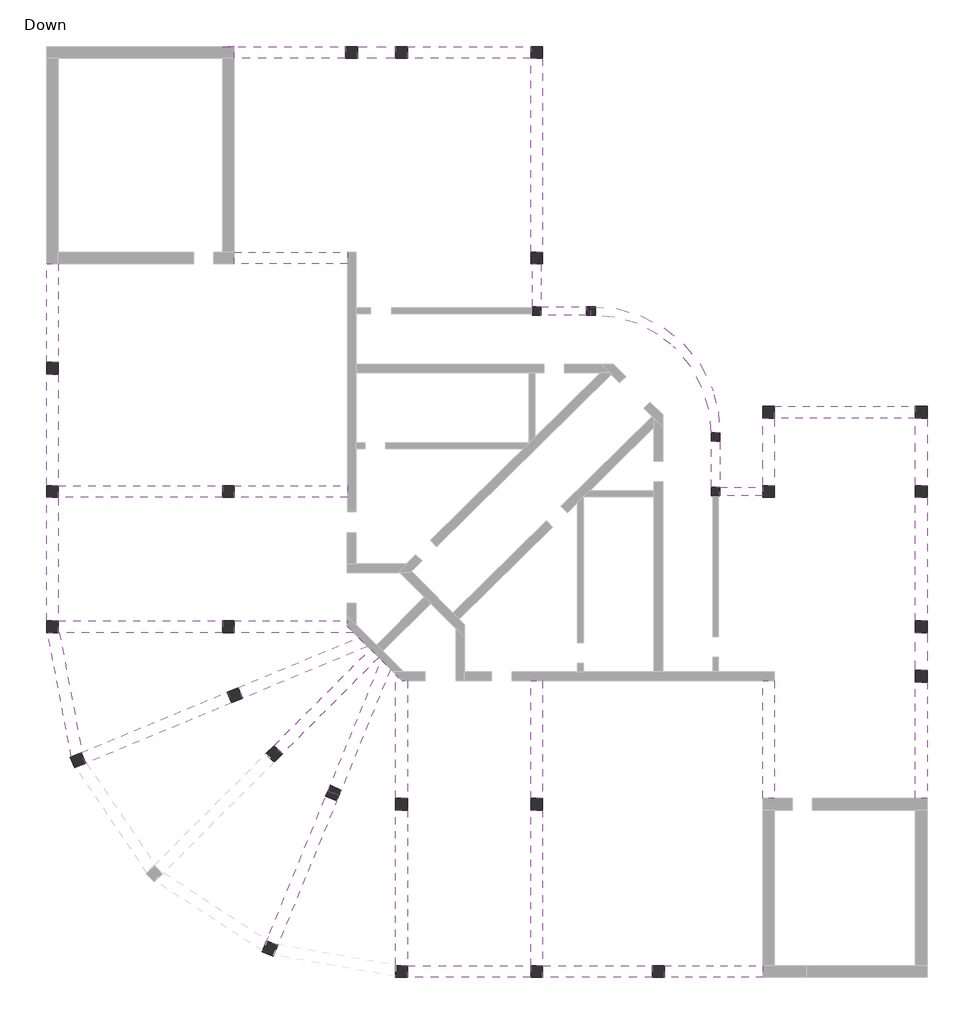
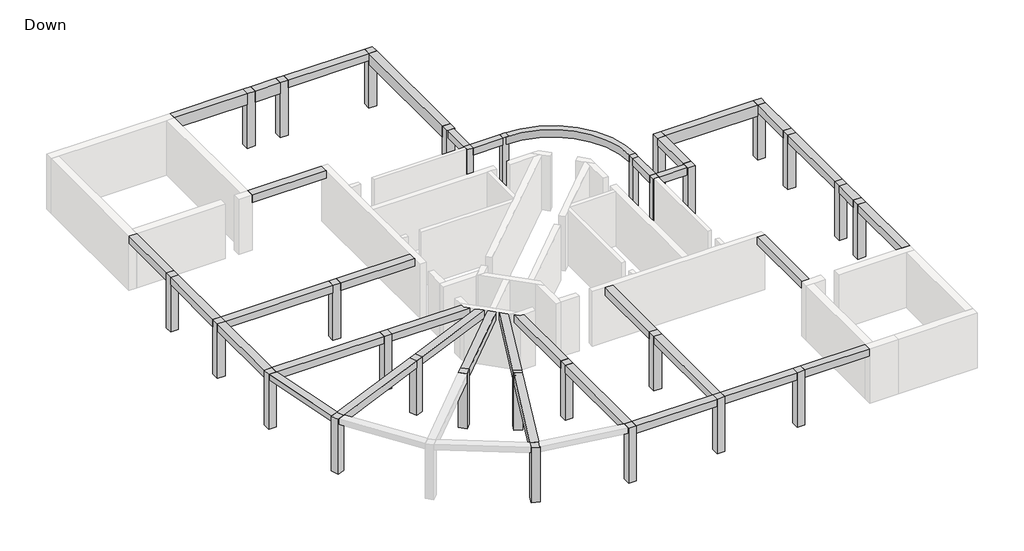
# One storey, part 2 of 2: 37 beams, 29 columns.
"""IFC4 building model written with IfcOpenShell, lengths in millimetres."""

from ifc_helpers import new_model, si_unit, point, frame, frame_2d, origin, origin_with_axes, place, context, project, spatial, polyline, circle_curve, trimmed, segment, composite_curve, outline, extrude, faceted_brep, element, save

model = new_model("IFC4")

# Units and contexts
model_context = context("Model", 3, world=origin())
ifc_project = project(units=[si_unit("LENGTHUNIT", "METRE", prefix="MILLI")], contexts=[model_context])

# Site, building, storey
site = spatial("IfcSite", under=ifc_project)
building = spatial("IfcBuilding", under=site)
storey = spatial("IfcBuildingStorey", under=building, Name="Down", Elevation=0.0)

# Beams
placement = place(None, origin())
element("IfcBeam", 1, ObjectType="Concrete Rectengular Beam : 30/40", at=placement, inside=storey, context=model_context, shape_type="Brep", body=[
    faceted_brep([(9669.6339123, 9562.1590026, 3000.0), (9669.6339123, 9862.1590026, 3000.0), (8219.6339123, 9862.1590026, 3000.0), (8219.6339123, 9562.1590026, 3000.0), (9669.6339123, 9862.1590026, 2600.0), (8219.6339123, 9862.1590026, 2600.0), (9669.6339123, 9562.1590026, 2600.0), (8219.6339123, 9562.1590026, 2600.0), (8219.6339123, 9562.1590026, 2800.0), (9669.6339123, 9562.1590026, 2800.0)], [[[0, 1, 2, 3]], [[1, 4, 5, 2]], [[4, 6, 7, 5]], [[0, 3, 8, 7, 6, 9]], [[4, 1, 0, 9, 6]], [[3, 2, 5, 7, 8]]]),
])
element("IfcBeam", 2, ObjectType="Concrete Rectengular Beam : 30/40", at=placement, inside=storey, context=model_context, shape_type="Brep", body=[
    faceted_brep([(7919.6339123, 9862.1590026, 3000.0), (8219.6339123, 9862.1590026, 3000.0), (8219.6339123, 11415.5910733, 3000.0), (7919.6339123, 11415.5910733, 3000.0), (8219.6339123, 9862.1590026, 2600.0), (8219.6339123, 11415.5910733, 2600.0), (7919.6339123, 9862.1590026, 2600.0), (7919.6339123, 11415.5910733, 2600.0), (7919.6339123, 11415.5910733, 2800.0), (7919.6339123, 9862.1590026, 2800.0)], [[[0, 1, 2, 3]], [[1, 4, 5, 2]], [[4, 6, 7, 5]], [[0, 3, 8, 7, 6, 9]], [[4, 1, 0, 9, 6]], [[3, 2, 5, 7, 8]]]),
])
element("IfcBeam", 3, ObjectType="Concrete Rectengular Beam : 30/40", at=placement, inside=storey, context=model_context, shape_type="SweptSolid", body=[
    extrude(outline(composite_curve([segment(polyline([(3827.8442558, 15704.0519912), (3819.9226923, 16003.9473877)]), True, "CONTINUOUS"), segment(trimmed(circle_curve(frame_2d((3933.1798389, 11716.2462427)), 4289.1966953), [point((3819.9226923, 16003.9473877))], [point((8219.6339123, 11562.8846875))], False, "CARTESIAN"), True, "CONTINUOUS"), segment(polyline([(8219.6339123, 11562.8846875), (8219.6339123, 11715.5910733), (7922.3764803, 11715.5910733)]), True, "CONTINUOUS"), segment(trimmed(circle_curve(frame_2d((3933.1798389, 11716.2462427)), 3989.1966953), [point((7922.3764803, 11715.5910733))], [point((3827.8442558, 15704.0519912))], True, "CARTESIAN"), True, "CONTINUOUS")], self_intersect=False)), frame((0.0, 0.0, 2600.0), z_axis=(0.0, 0.0, 1.0), x_axis=(1.0, 0.0, 0.0)), (0.0, 0.0, 1.0), 400.0),
])
element("IfcBeam", 4, ObjectType="Concrete Rectengular Beam : 30/40", at=placement, inside=storey, context=model_context, shape_type="Brep", body=[
    faceted_brep([(2129.020722, 16003.9996895, 3000.0), (2129.020722, 15703.9996895, 3000.0), (3673.883474, 15703.9996895, 3000.0), (3673.883474, 16003.9996895, 3000.0), (2129.020722, 16003.9996895, 2600.0), (3673.883474, 16003.9996895, 2600.0), (2129.020722, 15703.9996895, 2600.0), (3673.883474, 15703.9996895, 2600.0), (2129.020722, 15703.9996895, 2800.0), (3673.883474, 15703.9996895, 2800.0)], [[[0, 1, 2, 3]], [[4, 0, 3, 5]], [[6, 4, 5, 7]], [[2, 1, 8, 6, 7, 9]], [[1, 0, 4, 6, 8]], [[3, 2, 9, 7, 5]]]),
])
element("IfcBeam", 5, ObjectType="Concrete Rectengular Beam : 30/40", at=placement, inside=storey, context=model_context, shape_type="Brep", body=[
    faceted_brep([(2129.020722, 17453.6134053, 3000.0), (1829.020722, 17453.6134053, 3000.0), (1829.020722, 16003.9996895, 3000.0), (2129.020722, 16003.9996895, 3000.0), (2129.020722, 17453.6134053, 2600.0), (2129.020722, 16003.9996895, 2600.0), (1829.020722, 17453.6134053, 2600.0), (1829.020722, 16003.9996895, 2600.0), (1829.020722, 17453.6134053, 2800.0)], [[[0, 1, 2, 3]], [[4, 0, 3, 5]], [[6, 4, 5, 7]], [[1, 8, 6, 7, 2]], [[1, 0, 4, 6, 8]], [[2, 7, 5, 3]]]),
])
element("IfcBeam", 6, ObjectType="Concrete Rectengular Beam : 39/30", at=placement, inside=storey, context=model_context, shape_type="Brep", body=[
    faceted_brep([(-13852.0238981, 697.9157956, 3000.0), (-13520.7080657, 835.1736918, 3000.0), (-13484.0892311, 850.3441838, 3000.0), (-14261.3814687, 4919.511412, 3000.0), (-14296.6369988, 4919.511412, 3000.0), (-14658.4330031, 4919.511412, 3000.0), (-13484.0892311, 850.3441838, 2800.0), (-13484.0892311, 850.3441838, 2700.0), (-14261.3814687, 4919.511412, 2700.0), (-14261.3814687, 4919.511412, 2800.0), (-13852.0238981, 697.9157956, 2700.0), (-14658.4330031, 4919.511412, 2700.0)], [[[0, 1, 2, 3, 4, 5]], [[3, 2, 6, 7, 8, 9]], [[7, 10, 11, 8]], [[10, 0, 5, 11]], [[0, 10, 7, 6, 2, 1]], [[11, 5, 4, 3, 9, 8]]]),
])
element("IfcBeam", 7, ObjectType="Concrete Rectengular Beam : 40/40", at=placement, inside=storey, context=model_context, shape_type="Brep", body=[
    faceted_brep([(-2413.8658054, -6410.076772, 3000.0), (-2413.8658054, -6810.076772, 3000.0), (1779.020722, -6810.076772, 3000.0), (1779.020722, -6410.076772, 3000.0), (-2413.8658054, -6810.076772, 2600.0), (1779.020722, -6810.076772, 2600.0), (-2413.8658054, -6410.076772, 2600.0), (1779.020722, -6410.076772, 2600.0), (-2413.8658054, -6410.076772, 2800.0), (1779.020722, -6410.076772, 2800.0)], [[[0, 1, 2, 3]], [[1, 4, 5, 2]], [[4, 6, 7, 5]], [[6, 8, 0, 3, 9, 7]], [[1, 0, 8, 6, 4]], [[3, 2, 5, 7, 9]]]),
])
element("IfcBeam", 8, ObjectType="Concrete Rectengular Beam : 40/40", at=placement, inside=storey, context=model_context, shape_type="Brep", body=[
    faceted_brep([(2179.020722, -6410.076772, 3000.0), (2179.020722, -6810.076772, 3000.0), (5922.4147884, -6810.076772, 3000.0), (5922.4147884, -6410.076772, 3000.0), (2179.020722, -6810.076772, 2600.0), (5922.4147884, -6810.076772, 2600.0), (2179.020722, -6410.076772, 2600.0), (5922.4147884, -6410.076772, 2600.0), (2179.020722, -6410.076772, 2800.0)], [[[0, 1, 2, 3]], [[1, 4, 5, 2]], [[4, 6, 7, 5]], [[6, 8, 0, 3, 7]], [[1, 0, 8, 6, 4]], [[3, 2, 5, 7]]]),
])
element("IfcBeam", 9, ObjectType="Concrete Rectengular Beam : 40/40", at=placement, inside=storey, context=model_context, shape_type="Brep", body=[
    faceted_brep([(6322.4147884, -6410.076772, 3000.0), (6322.4147884, -6810.076772, 3000.0), (9669.6339123, -6810.076772, 3000.0), (9669.6339123, -6410.076772, 3000.0), (6322.4147884, -6810.076772, 2600.0), (9669.6339123, -6810.076772, 2600.0), (6322.4147884, -6410.076772, 2600.0), (9669.6339123, -6410.076772, 2600.0), (9669.6339123, -6410.076772, 2800.0)], [[[0, 1, 2, 3]], [[1, 4, 5, 2]], [[4, 6, 7, 5]], [[6, 0, 3, 8, 7]], [[1, 0, 6, 4]], [[3, 2, 5, 7, 8]]]),
])
element("IfcBeam", 10, ObjectType="Concrete Rectengular Beam : 40/40", at=placement, inside=storey, context=model_context, shape_type="Brep", body=[
    faceted_brep([(1779.020722, -6410.076772, 3000.0), (2179.020722, -6410.076772, 3000.0), (2179.020722, -1123.2844162, 3000.0), (1779.020722, -1123.2844162, 3000.0), (2179.020722, -6410.076772, 2800.0), (2179.020722, -6410.076772, 2600.0), (2179.020722, -1123.2844162, 2600.0), (1779.020722, -6410.076772, 2600.0), (1779.020722, -1123.2844162, 2600.0), (1779.020722, -6410.076772, 2800.0)], [[[0, 1, 2, 3]], [[1, 4, 5, 6, 2]], [[5, 7, 8, 6]], [[7, 9, 0, 3, 8]], [[0, 9, 7, 5, 4, 1]], [[3, 2, 6, 8]]]),
])
element("IfcBeam", 11, ObjectType="Concrete Rectengular Beam : 40/40", at=placement, inside=storey, context=model_context, shape_type="Brep", body=[
    faceted_brep([(1779.020722, -723.2844162, 3000.0), (2179.020722, -723.2844162, 3000.0), (2179.020722, 3279.3391577, 3000.0), (1779.020722, 3279.3391577, 3000.0), (2179.020722, -723.2844162, 2600.0), (2179.020722, 3279.3391577, 2600.0), (2179.020722, 3279.3391577, 2800.0), (1779.020722, -723.2844162, 2600.0), (1779.020722, 3279.3391577, 2600.0), (1779.020722, 3279.3391577, 2800.0)], [[[0, 1, 2, 3]], [[1, 4, 5, 6, 2]], [[4, 7, 8, 5]], [[7, 0, 3, 9, 8]], [[1, 0, 7, 4]], [[3, 2, 6, 5, 8, 9]]]),
])
element("IfcBeam", 12, ObjectType="Concrete Rectengular Beam : 40/40", at=placement, inside=storey, context=model_context, shape_type="Brep", body=[
    faceted_brep([(-2813.8658054, -6410.076772, 3000.0), (-2413.8658054, -6410.076772, 3000.0), (-2413.8658054, -1123.2844162, 3000.0), (-2813.8658054, -1123.2844162, 3000.0), (-2813.8658054, -6379.2217224, 3000.0), (-2413.8658054, -6410.076772, 2800.0), (-2413.8658054, -6410.076772, 2600.0), (-2413.8658054, -1123.2844162, 2600.0), (-2813.8658054, -6410.076772, 2600.0), (-2813.8658054, -1123.2844162, 2600.0)], [[[0, 1, 2, 3, 4]], [[1, 5, 6, 7, 2]], [[6, 8, 9, 7]], [[8, 0, 4, 3, 9]], [[6, 5, 1, 0, 8]], [[3, 2, 7, 9]]]),
])
element("IfcBeam", 13, ObjectType="Concrete Rectengular Beam : 40/40", at=placement, inside=storey, context=model_context, shape_type="Brep", body=[
    faceted_brep([(-2413.8658054, -723.2844162, 3000.0), (-2413.8658054, -723.2844162, 2600.0), (-2413.8658054, 3279.3391577, 2600.0), (-2413.8658054, 3279.3391577, 2800.0), (-2413.8658054, 3279.3391577, 3000.0), (-2813.8658054, -723.2844162, 3000.0), (-2813.8658054, -723.2844162, 2600.0), (-2609.1120413, 3279.3391577, 2600.0), (-2609.1120413, 3279.3391577, 3000.0), (-2813.8658054, 3484.0929218, 2600.0), (-2813.8658054, 3484.0929218, 2800.0), (-2813.8658054, 3484.0929218, 3000.0)], [[[0, 1, 2, 3, 4]], [[0, 5, 6, 1]], [[7, 8, 4, 3, 2]], [[8, 7, 9, 10, 11]], [[5, 0, 4, 8, 11]], [[1, 6, 9, 7, 2]], [[6, 5, 11, 10, 9]]]),
])
element("IfcBeam", 14, ObjectType="Concrete Rectengular Beam : 40/40", at=placement, inside=storey, context=model_context, shape_type="Brep", body=[
    faceted_brep([(-4749.0136896, -620.4955799, 3000.0), (-5119.2358115, -469.0506048, 3000.0), (-5120.1129012, -471.1947368, 3000.0), (-5193.4008185, -650.3542517, 3000.0), (-7191.7801663, -5535.5889186, 3000.0), (-7204.9594265, -5567.8069151, 3000.0), (-6834.7373046, -5719.2518901, 3000.0), (-6818.4727302, -5679.49154, 3000.0), (-4750.6157411, -624.4119522, 3000.0), (-6834.7373046, -5719.2518901, 2600.0), (-4749.0136896, -620.4955799, 2600.0), (-4749.0136896, -620.4955799, 2800.0), (-5119.2358115, -469.0506048, 2600.0), (-7204.9594265, -5567.8069151, 2600.0), (-5119.2358115, -469.0506048, 2800.0)], [[[0, 1, 2, 3, 4, 5, 6, 7, 8]], [[9, 10, 11, 0, 8, 7, 6]], [[12, 10, 9, 13]], [[12, 13, 5, 4, 3, 2, 1, 14]], [[1, 0, 11, 10, 12, 14]], [[6, 5, 13, 9]]]),
])
element("IfcBeam", 15, ObjectType="Concrete Rectengular Beam : 40/40", at=placement, inside=storey, context=model_context, shape_type="Brep", body=[
    faceted_brep([(-5119.2358115, -469.0506048, 3000.0), (-4749.0136896, -620.4955799, 3000.0), (-4673.1767374, -435.1046991, 3000.0), (-2995.6201329, 3665.8472494, 3000.0), (-3302.3291451, 3972.5562616, 3000.0), (-4749.0136896, -620.4955799, 2800.0), (-4749.0136896, -620.4955799, 2600.0), (-2995.6201329, 3665.8472494, 2600.0), (-2995.6201329, 3665.8472494, 2800.0), (-5119.2358115, -469.0506048, 2600.0), (-3302.3291451, 3972.5562616, 2600.0), (-5119.2358115, -469.0506048, 2800.0), (-3302.3291451, 3972.5562616, 2800.0)], [[[0, 1, 2, 3, 4]], [[1, 5, 6, 7, 8, 3, 2]], [[6, 9, 10, 7]], [[9, 11, 0, 4, 12, 10]], [[9, 6, 5, 1, 0, 11]], [[4, 3, 8, 7, 10, 12]]]),
])
element("IfcBeam", 16, ObjectType="Concrete Rectengular Beam : 40/40", at=placement, inside=storey, context=model_context, shape_type="Brep", body=[
    faceted_brep([(-6954.3338626, 1076.4917444, 3000.0), (-6671.4911578, 793.6490243, 3000.0), (-3397.4447571, 4067.6718736, 3000.0), (-3680.2874696, 4350.514586, 3000.0), (-6671.4911578, 793.6490243, 2600.0), (-3397.4447571, 4067.6718736, 2600.0), (-3397.4447571, 4067.6718736, 2800.0), (-6954.3338626, 1076.4917444, 2600.0), (-3680.2874696, 4350.514586, 2600.0), (-3680.2874696, 4350.514586, 2800.0)], [[[0, 1, 2, 3]], [[1, 4, 5, 6, 2]], [[4, 7, 8, 5]], [[7, 0, 3, 9, 8]], [[1, 0, 7, 4]], [[3, 2, 6, 5, 8, 9]]]),
])
element("IfcBeam", 17, ObjectType="Concrete Rectengular Beam : 40/40", at=placement, inside=storey, context=model_context, shape_type="Brep", body=[
    faceted_brep([(-13520.7080657, 835.1736918, 3000.0), (-13367.6133817, 465.6307069, 3000.0), (-13331.7826338, 480.4747094, 3000.0), (-8393.9631353, 2526.1201326, 3000.0), (-8547.0578193, 2895.6631176, 3000.0), (-13484.0892311, 850.3441838, 3000.0), (-13367.6133817, 465.6307069, 2600.0), (-8393.9631353, 2526.1201326, 2600.0), (-8393.9631353, 2526.1201326, 2800.0), (-13520.7080657, 835.1736918, 2600.0), (-8547.0578193, 2895.6631176, 2600.0), (-8547.0578193, 2895.6631176, 2800.0)], [[[0, 1, 2, 3, 4, 5]], [[1, 6, 7, 8, 3, 2]], [[6, 9, 10, 7]], [[9, 0, 5, 4, 11, 10]], [[1, 0, 9, 6]], [[4, 3, 8, 7, 10, 11]]]),
])
element("IfcBeam", 18, ObjectType="Concrete Rectengular Beam : 40/40", at=placement, inside=storey, context=model_context, shape_type="Brep", body=[
    faceted_brep([(-8177.5148344, 3048.7578016, 3000.0), (-8024.4201504, 2679.2148167, 3000.0), (-3771.0702765, 4441.2973929, 3000.0), (-4077.2097101, 4747.4368266, 3000.0), (-8024.4201504, 2679.2148167, 2800.0), (-8024.4201504, 2679.2148167, 2600.0), (-3771.0702765, 4441.2973929, 2600.0), (-3771.0702765, 4441.2973929, 2800.0), (-8177.5148344, 3048.7578016, 2600.0), (-4077.2097101, 4747.4368266, 2600.0), (-8177.5148344, 3048.7578016, 2800.0), (-4077.2097101, 4747.4368266, 2800.0)], [[[0, 1, 2, 3]], [[1, 4, 5, 6, 7, 2]], [[5, 8, 9, 6]], [[8, 10, 0, 3, 11, 9]], [[1, 0, 10, 8, 5, 4]], [[3, 2, 7, 6, 9, 11]]]),
])
element("IfcBeam", 19, ObjectType="Concrete Rectengular Beam : 40/40", at=placement, inside=storey, context=model_context, shape_type="Brep", body=[
    faceted_brep([(-14296.6369988, 5319.511412, 3000.0), (-14296.6369988, 4919.511412, 3000.0), (-14261.3814687, 4919.511412, 3000.0), (-8707.7294598, 4919.511412, 3000.0), (-8707.7294598, 5319.511412, 3000.0), (-14296.6369988, 4919.511412, 2600.0), (-8707.7294598, 4919.511412, 2600.0), (-14296.6369988, 5319.511412, 2600.0), (-8707.7294598, 5319.511412, 2600.0), (-14296.6369988, 5319.511412, 2800.0)], [[[0, 1, 2, 3, 4]], [[1, 5, 6, 3, 2]], [[5, 7, 8, 6]], [[7, 9, 0, 4, 8]], [[1, 0, 9, 7, 5]], [[4, 3, 6, 8]]]),
])
element("IfcBeam", 20, ObjectType="Concrete Rectengular Beam : 40/40", at=placement, inside=storey, context=model_context, shape_type="Brep", body=[
    faceted_brep([(-8307.7294598, 5319.511412, 3000.0), (-8307.7294598, 4919.511412, 3000.0), (-4249.2842956, 4919.511412, 3000.0), (-4467.7621118, 5137.9892282, 3000.0), (-4467.7621118, 5319.511412, 3000.0), (-8307.7294598, 4919.511412, 2600.0), (-4249.2842956, 4919.511412, 2600.0), (-4249.2842956, 4919.511412, 2800.0), (-8307.7294598, 5319.511412, 2600.0), (-4467.7621118, 5319.511412, 2600.0), (-4467.7621118, 5137.9892282, 2600.0), (-4467.7621118, 5319.511412, 2800.0)], [[[0, 1, 2, 3, 4]], [[1, 5, 6, 7, 2]], [[5, 8, 9, 10, 6]], [[8, 0, 4, 11, 9]], [[1, 0, 8, 5]], [[10, 3, 2, 7, 6]], [[3, 10, 9, 11, 4]]]),
])
element("IfcBeam", 21, ObjectType="Concrete Rectengular Beam : 40/40", at=placement, inside=storey, context=model_context, shape_type="Brep", body=[
    faceted_brep([(-14696.6369988, 5319.511412, 3000.0), (-14296.6369988, 5319.511412, 3000.0), (-14296.6369988, 9512.1590026, 3000.0), (-14696.6369988, 9512.1590026, 3000.0), (-14296.6369988, 5319.511412, 2800.0), (-14296.6369988, 5319.511412, 2600.0), (-14296.6369988, 9512.1590026, 2600.0), (-14296.6369988, 9512.1590026, 2800.0), (-14696.6369988, 5319.511412, 2600.0), (-14696.6369988, 9512.1590026, 2600.0)], [[[0, 1, 2, 3]], [[1, 4, 5, 6, 7, 2]], [[5, 8, 9, 6]], [[8, 0, 3, 9]], [[5, 4, 1, 0, 8]], [[3, 2, 7, 6, 9]]]),
])
element("IfcBeam", 22, ObjectType="Concrete Rectengular Beam : 40/40", at=placement, inside=storey, context=model_context, shape_type="Brep", body=[
    faceted_brep([(-14296.6369988, 9912.1590026, 3000.0), (-14296.6369988, 9512.1590026, 3000.0), (-8707.7294598, 9512.1590026, 3000.0), (-8707.7294598, 9912.1590026, 3000.0), (-14296.6369988, 9512.1590026, 2800.0), (-14296.6369988, 9512.1590026, 2600.0), (-8707.7294598, 9512.1590026, 2600.0), (-14296.6369988, 9912.1590026, 2600.0), (-8707.7294598, 9912.1590026, 2600.0), (-14296.6369988, 9912.1590026, 2800.0)], [[[0, 1, 2, 3]], [[1, 4, 5, 6, 2]], [[5, 7, 8, 6]], [[7, 9, 0, 3, 8]], [[5, 4, 1, 0, 9, 7]], [[3, 2, 6, 8]]]),
])
element("IfcBeam", 23, ObjectType="Concrete Rectengular Beam : 40/40", at=placement, inside=storey, context=model_context, shape_type="Brep", body=[
    faceted_brep([(-14696.6369988, 9912.1590026, 3000.0), (-14296.6369988, 9912.1590026, 3000.0), (-14296.6369988, 13707.3138675, 3000.0), (-14696.6369988, 13707.3138675, 3000.0), (-14296.6369988, 9912.1590026, 2800.0), (-14296.6369988, 9912.1590026, 2600.0), (-14296.6369988, 13707.3138675, 2600.0), (-14696.6369988, 9912.1590026, 2600.0), (-14696.6369988, 13707.3138675, 2600.0)], [[[0, 1, 2, 3]], [[1, 4, 5, 6, 2]], [[5, 7, 8, 6]], [[7, 0, 3, 8]], [[5, 4, 1, 0, 7]], [[3, 2, 6, 8]]]),
])
element("IfcBeam", 24, ObjectType="Concrete Rectengular Beam : 40/40", at=placement, inside=storey, context=model_context, shape_type="Brep", body=[
    faceted_brep([(-14696.6369988, 14107.3138675, 3000.0), (-14296.6369988, 14107.3138675, 3000.0), (-14296.6369988, 17456.8664083, 3000.0), (-14696.6369988, 17456.8664083, 3000.0), (-14296.6369988, 14107.3138675, 2600.0), (-14296.6369988, 17456.8664083, 2600.0), (-14296.6369988, 17456.8664083, 2800.0), (-14696.6369988, 14107.3138675, 2600.0), (-14696.6369988, 17456.8664083, 2600.0)], [[[0, 1, 2, 3]], [[1, 4, 5, 6, 2]], [[4, 7, 8, 5]], [[7, 0, 3, 8]], [[1, 0, 7, 4]], [[3, 2, 6, 5, 8]]]),
])
element("IfcBeam", 25, ObjectType="Concrete Rectengular Beam : 40/40", at=placement, inside=storey, context=model_context, shape_type="Brep", body=[
    faceted_brep([(-8307.7294598, 9912.1590026, 3000.0), (-8307.7294598, 9512.1590026, 3000.0), (-4461.7067397, 9512.1590026, 3000.0), (-4461.7067397, 9912.1590026, 3000.0), (-8307.7294598, 9512.1590026, 2600.0), (-4461.7067397, 9512.1590026, 2600.0), (-4461.7067397, 9512.1590026, 2800.0), (-8307.7294598, 9912.1590026, 2600.0), (-4461.7067397, 9912.1590026, 2600.0), (-4461.7067397, 9912.1590026, 2800.0)], [[[0, 1, 2, 3]], [[1, 4, 5, 6, 2]], [[4, 7, 8, 5]], [[7, 0, 3, 9, 8]], [[1, 0, 7, 4]], [[3, 2, 6, 5, 8, 9]]]),
])
element("IfcBeam", 26, ObjectType="Concrete Rectengular Beam : 40/40", at=placement, inside=storey, context=model_context, shape_type="Brep", body=[
    faceted_brep([(15262.3806142, 3228.4489922, 3000.0), (14862.3806142, 3228.4489922, 3000.0), (14862.3806142, -716.1309652, 3000.0), (15262.3806142, -716.1309652, 3000.0), (15262.3806142, 3228.4489922, 2600.0), (15262.3806142, -716.1309652, 2600.0), (14862.3806142, 3228.4489922, 2600.0), (14862.3806142, -716.1309652, 2600.0), (14862.3806142, -716.1309652, 2800.0)], [[[0, 1, 2, 3]], [[4, 0, 3, 5]], [[6, 4, 5, 7]], [[1, 6, 7, 8, 2]], [[1, 0, 4, 6]], [[3, 2, 8, 7, 5]]]),
])
element("IfcBeam", 27, ObjectType="Concrete Rectengular Beam : 40/40", at=placement, inside=storey, context=model_context, shape_type="SweptSolid", body=[
    extrude(outline(polyline([(15262.3806142, 3628.4489922), (14862.3806142, 3628.4489922), (14862.3806142, 4919.511412), (15262.3806142, 4919.511412), (15262.3806142, 3628.4489922)])), frame((0.0, 0.0, 2600.0), z_axis=(0.0, 0.0, 1.0), x_axis=(1.0, 0.0, 0.0)), (0.0, 0.0, 1.0), 400.0),
])
element("IfcBeam", 28, ObjectType="Concrete Rectengular Beam : 40/40", at=placement, inside=storey, context=model_context, shape_type="SweptSolid", body=[
    extrude(outline(polyline([(15262.3806142, 5319.511412), (14862.3806142, 5319.511412), (14862.3806142, 9512.1590026), (15262.3806142, 9512.1590026), (15262.3806142, 5319.511412)])), frame((0.0, 0.0, 2600.0), z_axis=(0.0, 0.0, 1.0), x_axis=(1.0, 0.0, 0.0)), (0.0, 0.0, 1.0), 400.0),
])
element("IfcBeam", 29, ObjectType="Concrete Rectengular Beam : 40/40", at=placement, inside=storey, context=model_context, shape_type="Brep", body=[
    faceted_brep([(14862.3806142, 9912.1590026, 3000.0), (15262.3806142, 9912.1590026, 3000.0), (15262.3806142, 12213.3492909, 3000.0), (14862.3806142, 12213.3492909, 3000.0), (15262.3806142, 9912.1590026, 2600.0), (15262.3806142, 12213.3492909, 2600.0), (14862.3806142, 9912.1590026, 2600.0), (14862.3806142, 12213.3492909, 2600.0), (14862.3806142, 12213.3492909, 2800.0)], [[[0, 1, 2, 3]], [[1, 4, 5, 2]], [[4, 6, 7, 5]], [[6, 0, 3, 8, 7]], [[1, 0, 6, 4]], [[3, 2, 5, 7, 8]]]),
])
element("IfcBeam", 30, ObjectType="Concrete Rectengular Beam : 40/40", at=placement, inside=storey, context=model_context, shape_type="Brep", body=[
    faceted_brep([(10069.6339123, 12213.3492909, 3000.0), (9669.6339123, 12213.3492909, 3000.0), (9669.6339123, 9912.1590026, 3000.0), (10069.6339123, 9912.1590026, 3000.0), (10069.6339123, 9912.1590026, 2800.0), (10069.6339123, 9912.1590026, 2600.0), (10069.6339123, 12213.3492909, 2600.0), (10069.6339123, 12213.3492909, 2800.0), (9669.6339123, 12213.3492909, 2600.0), (9669.6339123, 9912.1590026, 2600.0)], [[[0, 1, 2, 3]], [[0, 3, 4, 5, 6, 7]], [[8, 6, 5, 9]], [[1, 8, 9, 2]], [[1, 0, 7, 6, 8]], [[3, 2, 9, 5, 4]]]),
])
element("IfcBeam", 31, ObjectType="Concrete Rectengular Beam : 40/40", at=placement, inside=storey, context=model_context, shape_type="Brep", body=[
    faceted_brep([(1779.020722, 24445.393344, 3000.0), (1779.020722, 24845.393344, 3000.0), (-2413.8658054, 24845.393344, 3000.0), (-2413.8658054, 24445.393344, 3000.0), (1779.020722, 24845.393344, 2600.0), (-2413.8658054, 24845.393344, 2600.0), (1779.020722, 24445.393344, 2600.0), (-2413.8658054, 24445.393344, 2600.0), (1779.020722, 24445.393344, 2800.0)], [[[0, 1, 2, 3]], [[1, 4, 5, 2]], [[4, 6, 7, 5]], [[6, 8, 0, 3, 7]], [[0, 8, 6, 4, 1]], [[3, 2, 5, 7]]]),
])
element("IfcBeam", 32, ObjectType="Concrete Rectengular Beam : 40/40", at=placement, inside=storey, context=model_context, shape_type="Brep", body=[
    faceted_brep([(-8305.861308, 17856.8664083, 3000.0), (-8305.861308, 17456.8664083, 3000.0), (-4461.7067397, 17456.8664083, 3000.0), (-4461.7067397, 17856.8664083, 3000.0), (-8305.861308, 17856.8664083, 2600.0), (-8305.861308, 17856.8664083, 2800.0), (-4461.7067397, 17856.8664083, 2600.0), (-8305.861308, 17456.8664083, 2600.0), (-4461.7067397, 17456.8664083, 2600.0), (-4461.7067397, 17456.8664083, 2800.0)], [[[0, 1, 2, 3]], [[4, 5, 0, 3, 6]], [[7, 4, 6, 8]], [[1, 7, 8, 9, 2]], [[1, 0, 5, 4, 7]], [[3, 2, 9, 8, 6]]]),
])
element("IfcBeam", 33, ObjectType="Concrete Rectengular Beam : 40/40", at=placement, inside=storey, context=model_context, shape_type="Brep", body=[
    faceted_brep([(10069.6339123, -716.1309652, 3000.0), (10069.6339123, 3279.3391577, 3000.0), (9669.6339123, 3279.3391577, 3000.0), (9669.6339123, -716.1309652, 3000.0), (10069.6339123, -716.1309652, 2800.0), (10069.6339123, -716.1309652, 2600.0), (10069.6339123, 3279.3391577, 2600.0), (9669.6339123, 3279.3391577, 2600.0), (9669.6339123, -716.1309652, 2600.0), (9669.6339123, 3279.3391577, 2800.0)], [[[0, 1, 2, 3]], [[1, 0, 4, 5, 6]], [[7, 6, 5, 8]], [[2, 9, 7, 8, 3]], [[2, 1, 6, 7, 9]], [[0, 3, 8, 5, 4]]]),
])
element("IfcBeam", 34, ObjectType="Concrete Rectengular Beam : 40/60", at=placement, inside=storey, context=model_context, shape_type="Brep", body=[
    faceted_brep([(14862.3806142, 12213.3492909, 3000.0), (14862.3806142, 12613.3492909, 3000.0), (10069.6339123, 12613.3492909, 3000.0), (10069.6339123, 12213.3492909, 3000.0), (14862.3806142, 12213.3492909, 2400.0), (14862.3806142, 12213.3492909, 2800.0), (10069.6339123, 12213.3492909, 2800.0), (10069.6339123, 12213.3492909, 2400.0), (14862.3806142, 12613.3492909, 2400.0), (10069.6339123, 12613.3492909, 2400.0)], [[[0, 1, 2, 3]], [[4, 5, 0, 3, 6, 7]], [[8, 4, 7, 9]], [[1, 8, 9, 2]], [[1, 0, 5, 4, 8]], [[3, 2, 9, 7, 6]]]),
])
element("IfcBeam", 35, ObjectType="Concrete Rectengular Beam : 40/60", at=placement, inside=storey, context=model_context, shape_type="Brep", body=[
    faceted_brep([(2179.020722, 24445.393344, 3000.0), (1779.020722, 24445.393344, 3000.0), (1779.020722, 17856.8664083, 3000.0), (1779.020722, 17853.6134053, 3000.0), (2179.020722, 17853.6134053, 3000.0), (2179.020722, 24445.393344, 2400.0), (2179.020722, 17853.6134053, 2400.0), (1779.020722, 24445.393344, 2400.0), (1779.020722, 17853.6134053, 2400.0), (1779.020722, 17853.6134053, 2800.0), (1779.020722, 24445.393344, 2800.0)], [[[0, 1, 2, 3, 4]], [[5, 0, 4, 6]], [[7, 5, 6, 8]], [[7, 8, 9, 3, 2, 1, 10]], [[1, 0, 5, 7, 10]], [[4, 3, 9, 8, 6]]]),
])
element("IfcBeam", 36, ObjectType="Concrete Rectengular Beam : 40/60", at=placement, inside=storey, context=model_context, shape_type="SweptSolid", body=[
    extrude(outline(polyline([(-2813.8658054, 24845.393344), (-2813.8658054, 24445.393344), (-4118.3634455, 24445.393344), (-4118.3634455, 24845.393344), (-2813.8658054, 24845.393344)])), frame((0.0, 0.0, 2400.0), z_axis=(0.0, 0.0, 1.0), x_axis=(1.0, 0.0, 0.0)), (0.0, 0.0, 1.0), 600.0),
])
element("IfcBeam", 37, ObjectType="Concrete Rectengular Beam : 40/60", at=placement, inside=storey, context=model_context, shape_type="Brep", body=[
    faceted_brep([(-4518.3634455, 24445.393344, 3000.0), (-4518.3634455, 24845.393344, 3000.0), (-8705.861308, 24845.393344, 3000.0), (-8705.861308, 24844.3058567, 3000.0), (-8305.861308, 24844.3058567, 3000.0), (-8305.861308, 24445.393344, 3000.0), (-4518.3634455, 24845.393344, 2400.0), (-8705.861308, 24845.393344, 2400.0), (-4518.3634455, 24445.393344, 2400.0), (-8305.861308, 24445.393344, 2400.0), (-8305.861308, 24844.3058567, 2400.0), (-8705.861308, 24844.3058567, 2400.0), (-8305.861308, 24445.393344, 2800.0)], [[[0, 1, 2, 3, 4, 5]], [[1, 6, 7, 2]], [[6, 8, 9, 10, 11, 7]], [[8, 0, 5, 12, 9]], [[1, 0, 8, 6]], [[2, 7, 11, 3]], [[10, 4, 3, 11]], [[4, 10, 9, 12, 5]]]),
])

# Columns
element("IfcColumn", 38, ObjectType="Concrete Rectengular Column : 30/30", at=placement, inside=storey, context=model_context, shape_type="Brep", body=[
    faceted_brep([(8219.6339123, 9862.1590026, 0.0), (8219.6339123, 9562.1590026, 0.0), (8168.0773416, 9562.1590026, 0.0), (7968.0773416, 9562.1590026, 0.0), (7919.6339123, 9562.1590026, 0.0), (7919.6339123, 9862.1590026, 0.0), (8219.6339123, 9862.1590026, 3000.0), (8219.6339123, 9562.1590026, 3000.0), (8219.6339123, 9562.1590026, 2600.0), (8219.6339123, 9862.1590026, 2600.0), (8168.0773416, 9562.1590026, 3000.0), (7968.0773416, 9562.1590026, 3000.0), (7919.6339123, 9562.1590026, 3000.0), (7919.6339123, 9562.1590026, 2800.0), (7919.6339123, 9862.1590026, 3000.0)], [[[0, 1, 2, 3, 4, 5]], [[6, 7, 8, 1, 0, 9]], [[7, 10, 11, 12, 13, 4, 3, 2, 1, 8]], [[12, 14, 5, 4, 13]], [[14, 6, 9, 0, 5]], [[6, 14, 12, 11, 10, 7]]]),
])
element("IfcColumn", 39, ObjectType="Concrete Rectengular Column : 30/30", at=placement, inside=storey, context=model_context, shape_type="SweptSolid", body=[
    extrude(outline(polyline([(8219.6339123, 11715.5910733), (8219.6339123, 11415.5910733), (7919.6339123, 11415.5910733), (7919.6339123, 11715.5910733), (8219.6339123, 11715.5910733)])), origin_with_axes(), (0.0, 0.0, 1.0), 3000.0),
])
element("IfcColumn", 40, ObjectType="Concrete Rectengular Column : 30/30", at=placement, inside=storey, context=model_context, shape_type="Brep", body=[
    faceted_brep([(2129.020722, 16003.9996895, 0.0), (2129.020722, 15703.9996895, 0.0), (1829.020722, 15703.9996895, 0.0), (1829.020722, 15761.3377606, 0.0), (1829.020722, 15961.3377606, 0.0), (1829.020722, 16003.9996895, 0.0), (2129.020722, 16003.9996895, 3000.0), (2129.020722, 15703.9996895, 3000.0), (1829.020722, 15703.9996895, 3000.0), (1829.020722, 15703.9996895, 2800.0), (1829.020722, 15761.3377606, 3000.0), (1829.020722, 15961.3377606, 3000.0), (1829.020722, 16003.9996895, 3000.0)], [[[0, 1, 2, 3, 4, 5]], [[6, 7, 1, 0]], [[7, 8, 9, 2, 1]], [[8, 10, 11, 12, 5, 4, 3, 2, 9]], [[12, 6, 0, 5]], [[6, 12, 11, 10, 8, 7]]]),
])
element("IfcColumn", 41, ObjectType="Concrete Rectengular Column : 30/30", at=placement, inside=storey, context=model_context, shape_type="SweptSolid", body=[
    extrude(outline(polyline([(3973.883474, 16003.9996895), (3973.883474, 15703.9996895), (3673.883474, 15703.9996895), (3673.883474, 16003.9996895), (3973.883474, 16003.9996895)])), origin_with_axes(), (0.0, 0.0, 1.0), 3000.0),
])
element("IfcColumn", 42, ObjectType="Concrete Rectengular Column : 40/40", at=placement, inside=storey, context=model_context, shape_type="SweptSolid", body=[
    extrude(outline(polyline([(-2413.8658054, -6410.076772), (-2413.8658054, -6810.076772), (-2813.8658054, -6810.076772), (-2813.8658054, -6410.076772), (-2413.8658054, -6410.076772)])), origin_with_axes(), (0.0, 0.0, 1.0), 3000.0),
])
element("IfcColumn", 43, ObjectType="Concrete Rectengular Column : 40/40", at=placement, inside=storey, context=model_context, shape_type="SweptSolid", body=[
    extrude(outline(polyline([(2179.020722, -6410.076772), (2179.020722, -6810.076772), (1779.020722, -6810.076772), (1779.020722, -6410.076772), (2179.020722, -6410.076772)])), origin_with_axes(), (0.0, 0.0, 1.0), 3000.0),
])
element("IfcColumn", 44, ObjectType="Concrete Rectengular Column : 40/40", at=placement, inside=storey, context=model_context, shape_type="SweptSolid", body=[
    extrude(outline(polyline([(6322.4147884, -6410.076772), (6322.4147884, -6810.076772), (5922.4147884, -6810.076772), (5922.4147884, -6410.076772), (6322.4147884, -6410.076772)])), origin_with_axes(), (0.0, 0.0, 1.0), 3000.0),
])
element("IfcColumn", 45, ObjectType="Concrete Rectengular Column : 40/40", at=placement, inside=storey, context=model_context, shape_type="SweptSolid", body=[
    extrude(outline(polyline([(-2413.8658054, -723.2844162), (-2413.8658054, -1123.2844162), (-2813.8658054, -1123.2844162), (-2813.8658054, -723.2844162), (-2413.8658054, -723.2844162)])), origin_with_axes(), (0.0, 0.0, 1.0), 3000.0),
])
element("IfcColumn", 46, ObjectType="Concrete Rectengular Column : 40/40", at=placement, inside=storey, context=model_context, shape_type="SweptSolid", body=[
    extrude(outline(polyline([(2179.020722, -723.2844162), (2179.020722, -1123.2844162), (1779.020722, -1123.2844162), (1779.020722, -723.2844162), (2179.020722, -723.2844162)])), origin_with_axes(), (0.0, 0.0, 1.0), 3000.0),
])
element("IfcColumn", 47, ObjectType="Concrete Rectengular Column : 40/40", at=placement, inside=storey, context=model_context, shape_type="SweptSolid", body=[
    extrude(outline(polyline([(15262.3806142, 3628.4489922), (15262.3806142, 3228.4489922), (14862.3806142, 3228.4489922), (14862.3806142, 3628.4489922), (15262.3806142, 3628.4489922)])), origin_with_axes(), (0.0, 0.0, 1.0), 3000.0),
])
element("IfcColumn", 48, ObjectType="Concrete Rectengular Column : 40/40", at=placement, inside=storey, context=model_context, shape_type="SweptSolid", body=[
    extrude(outline(polyline([(15262.3806142, 5319.511412), (15262.3806142, 4919.511412), (14862.3806142, 4919.511412), (14862.3806142, 5319.511412), (15262.3806142, 5319.511412)])), origin_with_axes(), (0.0, 0.0, 1.0), 3000.0),
])
element("IfcColumn", 49, ObjectType="Concrete Rectengular Column : 40/40", at=placement, inside=storey, context=model_context, shape_type="SweptSolid", body=[
    extrude(outline(polyline([(15262.3806142, 9912.1590026), (15262.3806142, 9512.1590026), (14862.3806142, 9512.1590026), (14862.3806142, 9912.1590026), (15262.3806142, 9912.1590026)])), origin_with_axes(), (0.0, 0.0, 1.0), 3000.0),
])
element("IfcColumn", 50, ObjectType="Concrete Rectengular Column : 40/40", at=placement, inside=storey, context=model_context, shape_type="SweptSolid", body=[
    extrude(outline(polyline([(15262.3806142, 12613.3492909), (15262.3806142, 12213.3492909), (14862.3806142, 12213.3492909), (14862.3806142, 12613.3492909), (15262.3806142, 12613.3492909)])), origin_with_axes(), (0.0, 0.0, 1.0), 3000.0),
])
element("IfcColumn", 51, ObjectType="Concrete Rectengular Column : 40/40", at=placement, inside=storey, context=model_context, shape_type="SweptSolid", body=[
    extrude(outline(polyline([(10069.6339123, 12613.3492909), (10069.6339123, 12213.3492909), (9669.6339123, 12213.3492909), (9669.6339123, 12613.3492909), (10069.6339123, 12613.3492909)])), origin_with_axes(), (0.0, 0.0, 1.0), 3000.0),
])
element("IfcColumn", 52, ObjectType="Concrete Rectengular Column : 40/40", at=placement, inside=storey, context=model_context, shape_type="Brep", body=[
    faceted_brep([(10069.6339123, 9912.1590026, 0.0), (10069.6339123, 9512.1590026, 0.0), (9669.6339123, 9512.1590026, 0.0), (9669.6339123, 9912.1590026, 0.0), (10069.6339123, 9912.1590026, 3000.0), (10069.6339123, 9512.1590026, 3000.0), (10069.6339123, 9512.1590026, 2800.0), (9669.6339123, 9512.1590026, 3000.0), (9669.6339123, 9512.1590026, 2800.0), (9669.6339123, 9562.1590026, 3000.0), (9669.6339123, 9912.1590026, 3000.0)], [[[0, 1, 2, 3]], [[4, 5, 6, 1, 0]], [[5, 7, 8, 2, 1, 6]], [[7, 9, 10, 3, 2, 8]], [[10, 4, 0, 3]], [[4, 10, 9, 7, 5]]]),
])
element("IfcColumn", 53, ObjectType="Concrete Rectengular Column : 40/40", at=placement, inside=storey, context=model_context, shape_type="SweptSolid", body=[
    extrude(outline(polyline([(-13367.6133817, 465.6307069), (-13737.1563666, 312.5360228), (-13890.2510506, 682.0790078), (-13520.7080657, 835.1736918), (-13367.6133817, 465.6307069)])), origin_with_axes(), (0.0, 0.0, 1.0), 3000.0),
])
element("IfcColumn", 54, ObjectType="Concrete Rectengular Column : 40/40", at=placement, inside=storey, context=model_context, shape_type="SweptSolid", body=[
    extrude(outline(polyline([(-7204.9594265, -5567.8069151), (-6834.7373046, -5719.2518901), (-6986.1822797, -6089.474012), (-7356.4044016, -5938.0290369), (-7204.9594265, -5567.8069151)])), origin_with_axes(), (0.0, 0.0, 1.0), 3000.0),
])
element("IfcColumn", 55, ObjectType="Concrete Rectengular Column : 40/40", at=placement, inside=storey, context=model_context, shape_type="SweptSolid", body=[
    extrude(outline(polyline([(-14296.6369988, 5319.511412), (-14296.6369988, 4919.511412), (-14696.6369988, 4919.511412), (-14696.6369988, 5319.511412), (-14296.6369988, 5319.511412)])), origin_with_axes(), (0.0, 0.0, 1.0), 3000.0),
])
element("IfcColumn", 56, ObjectType="Concrete Rectengular Column : 40/40", at=placement, inside=storey, context=model_context, shape_type="SweptSolid", body=[
    extrude(outline(polyline([(-14296.6369988, 9912.1590026), (-14296.6369988, 9512.1590026), (-14696.6369988, 9512.1590026), (-14696.6369988, 9912.1590026), (-14296.6369988, 9912.1590026)])), origin_with_axes(), (0.0, 0.0, 1.0), 3000.0),
])
element("IfcColumn", 57, ObjectType="Concrete Rectengular Column : 40/40", at=placement, inside=storey, context=model_context, shape_type="SweptSolid", body=[
    extrude(outline(polyline([(-14296.6369988, 14107.3138675), (-14296.6369988, 13707.3138675), (-14696.6369988, 13707.3138675), (-14696.6369988, 14107.3138675), (-14296.6369988, 14107.3138675)])), origin_with_axes(), (0.0, 0.0, 1.0), 3000.0),
])
element("IfcColumn", 58, ObjectType="Concrete Rectengular Column : 40/40", at=placement, inside=storey, context=model_context, shape_type="SweptSolid", body=[
    extrude(outline(polyline([(-8307.7294598, 9912.1590026), (-8307.7294598, 9512.1590026), (-8707.7294598, 9512.1590026), (-8707.7294598, 9912.1590026), (-8307.7294598, 9912.1590026)])), origin_with_axes(), (0.0, 0.0, 1.0), 3000.0),
])
element("IfcColumn", 59, ObjectType="Concrete Rectengular Column : 40/40", at=placement, inside=storey, context=model_context, shape_type="SweptSolid", body=[
    extrude(outline(polyline([(2179.020722, 24845.393344), (2179.020722, 24445.393344), (1779.020722, 24445.393344), (1779.020722, 24845.393344), (2179.020722, 24845.393344)])), origin_with_axes(), (0.0, 0.0, 1.0), 3000.0),
])
element("IfcColumn", 60, ObjectType="Concrete Rectengular Column : 40/40", at=placement, inside=storey, context=model_context, shape_type="SweptSolid", body=[
    extrude(outline(polyline([(-2413.8658054, 24845.393344), (-2413.8658054, 24445.393344), (-2813.8658054, 24445.393344), (-2813.8658054, 24845.393344), (-2413.8658054, 24845.393344)])), origin_with_axes(), (0.0, 0.0, 1.0), 3000.0),
])
element("IfcColumn", 61, ObjectType="Concrete Rectengular Column : 40/40", at=placement, inside=storey, context=model_context, shape_type="SweptSolid", body=[
    extrude(outline(polyline([(-4118.3634455, 24845.393344), (-4118.3634455, 24445.393344), (-4518.3634455, 24445.393344), (-4518.3634455, 24845.393344), (-4118.3634455, 24845.393344)])), origin_with_axes(), (0.0, 0.0, 1.0), 3000.0),
])
element("IfcColumn", 62, ObjectType="Concrete Rectengular Column : 40/40", at=placement, inside=storey, context=model_context, shape_type="Brep", body=[
    faceted_brep([(2179.020722, 17853.6134053, 0.0), (2179.020722, 17453.6134053, 0.0), (1779.020722, 17453.6134053, 0.0), (1779.020722, 17853.6134053, 0.0), (2179.020722, 17853.6134053, 3000.0), (2179.020722, 17453.6134053, 3000.0), (1829.020722, 17453.6134053, 3000.0), (1779.020722, 17453.6134053, 3000.0), (1779.020722, 17453.6134053, 2800.0), (1779.020722, 17853.6134053, 3000.0)], [[[0, 1, 2, 3]], [[4, 5, 1, 0]], [[5, 6, 7, 8, 2, 1]], [[7, 9, 3, 2, 8]], [[9, 4, 0, 3]], [[4, 9, 7, 6, 5]]]),
])
element("IfcColumn", 63, ObjectType="Concrete Rectengular Column : 40/40", at=placement, inside=storey, context=model_context, shape_type="Brep", body=[
    faceted_brep([(-5040.12681, -280.8809609, 0.0), (-4671.3715454, -435.8633948, 0.0), (-4826.3539793, -804.6186594, 0.0), (-5195.1092439, -649.6362255, 0.0), (-5040.12681, -280.8809609, 3000.0), (-4673.1767374, -435.1046991, 3000.0), (-4671.3715454, -435.8633948, 3000.0), (-4671.3715454, -435.8633948, 2800.0), (-4750.6157411, -624.4119522, 3000.0), (-4826.3539793, -804.6186594, 3000.0), (-5193.4008185, -650.3542517, 3000.0), (-5195.1092439, -649.6362255, 3000.0), (-5195.1092439, -649.6362255, 2800.0), (-5120.1129012, -471.1947368, 3000.0)], [[[0, 1, 2, 3]], [[4, 5, 6, 7, 1, 0]], [[6, 8, 9, 2, 1, 7]], [[9, 10, 11, 12, 3, 2]], [[11, 13, 4, 0, 3, 12]], [[4, 13, 11, 10, 9, 8, 6, 5]]]),
])
element("IfcColumn", 64, ObjectType="Concrete Rectengular Column : 40/40", at=placement, inside=storey, context=model_context, shape_type="SweptSolid", body=[
    extrude(outline(polyline([(-6671.4910949, 793.6489615), (-6954.333815, 510.8062567), (-7237.1765199, 793.6489768), (-6954.3337998, 1076.4916816), (-6671.4910949, 793.6489615)])), origin_with_axes(), (0.0, 0.0, 1.0), 3000.0),
])
element("IfcColumn", 65, ObjectType="Concrete Rectengular Column : 40/40", at=placement, inside=storey, context=model_context, shape_type="SweptSolid", body=[
    extrude(outline(polyline([(-8177.5148344, 3048.7578016), (-8024.4201504, 2679.2148167), (-8393.9631353, 2526.1201326), (-8547.0578193, 2895.6631176), (-8177.5148344, 3048.7578016)])), origin_with_axes(), (0.0, 0.0, 1.0), 3000.0),
])
element("IfcColumn", 66, ObjectType="Concrete Rectengular Column : 40/40", at=placement, inside=storey, context=model_context, shape_type="SweptSolid", body=[
    extrude(outline(polyline([(-8307.7294598, 5319.511412), (-8307.7294598, 4919.511412), (-8707.7294598, 4919.511412), (-8707.7294598, 5319.511412), (-8307.7294598, 5319.511412)])), origin_with_axes(), (0.0, 0.0, 1.0), 3000.0),
])

save(model, "model.ifc")

# Revit data of these elements
# Type "Concrete Rectengular Beam : 30/40"
#   Length [instance default] = 152.4 cm
#   b = 30 cm
#   h = 40 cm
#   Structural Material [instance default] = Concrete
#   Assembly Code = ""
# Type "Concrete Rectengular Beam : 39/30"
#   Length [instance default] = 152.4 cm
#   b = 39 cm
#   h = 30 cm
#   Structural Material [instance default] = Concrete
#   Assembly Code = ""
# Type "Concrete Rectengular Beam : 40/40"
#   Length [instance default] = 152.4 cm
#   b = 40 cm
#   h = 40 cm
#   Structural Material [instance default] = Concrete
#   Assembly Code = ""
# Type "Concrete Rectengular Beam : 40/60"
#   Length [instance default] = 152.4 cm
#   b = 40 cm
#   h = 60 cm
#   Structural Material [instance default] = Concrete
#   Assembly Code = ""
# Type "Concrete Rectengular Column : 30/30"
#   b = 30 cm
#   h = 30 cm
#   Structural Material [instance default] = Concrete
# Type "Concrete Rectengular Column : 40/40"
#   b = 40 cm
#   h = 40 cm
#   Structural Material [instance default] = Concrete
# Element 1 (IfcBeam, "Concrete Rectengular Beam : 30/40")
#   Comments = ""
#   Mark = "B1"
#   SOFiSTiK_AMG_Comments = ""
#   SOFiSTiK_AMG_Scheduled = yes
#   SOFiSTiK_AMG_Adjusted = yes
#   Structural Material = Concrete
#   Phase Created = New Construction
#   Materials on its faces: "Concrete"
# Element 2 (IfcBeam, "Concrete Rectengular Beam : 30/40")
#   Comments = ""
#   Mark = "B2"
#   SOFiSTiK_AMG_Comments = ""
#   SOFiSTiK_AMG_Scheduled = yes
#   SOFiSTiK_AMG_Adjusted = yes
#   Structural Material = Concrete
#   Phase Created = New Construction
#   Materials on its faces: "Concrete"
# Element 3 (IfcBeam, "Concrete Rectengular Beam : 30/40")
#   Comments = ""
#   Mark = "B3"
#   SOFiSTiK_AMG_Comments = "Not line-shaped /"
#   SOFiSTiK_AMG_Scheduled = yes
#   SOFiSTiK_AMG_Adjusted = no
#   Structural Material = Concrete
#   Phase Created = New Construction
#   Materials on its faces: "Concrete"
# Element 4 (IfcBeam, "Concrete Rectengular Beam : 30/40")
#   Comments = ""
#   Mark = "B4"
#   SOFiSTiK_AMG_Comments = ""
#   SOFiSTiK_AMG_Scheduled = yes
#   SOFiSTiK_AMG_Adjusted = yes
#   Structural Material = Concrete
#   Phase Created = New Construction
#   Materials on its faces: "Concrete"
# Element 5 (IfcBeam, "Concrete Rectengular Beam : 30/40")
#   Comments = ""
#   Mark = "B5"
#   SOFiSTiK_AMG_Comments = ""
#   SOFiSTiK_AMG_Scheduled = yes
#   SOFiSTiK_AMG_Adjusted = yes
#   Structural Material = Concrete
#   Phase Created = New Construction
#   Materials on its faces: "Concrete"
# Element 6 (IfcBeam, "Concrete Rectengular Beam : 39/30")
#   Comments = ""
#   Mark = "B8"
#   SOFiSTiK_AMG_Comments = ""
#   SOFiSTiK_AMG_Scheduled = yes
#   SOFiSTiK_AMG_Adjusted = yes
#   Structural Material = Concrete
#   Phase Created = New Construction
#   Materials on its faces: "Concrete"
# Element 7 (IfcBeam, "Concrete Rectengular Beam : 40/40")
#   Comments = ""
#   Mark = "B10"
#   SOFiSTiK_AMG_Comments = ""
#   SOFiSTiK_AMG_Scheduled = yes
#   SOFiSTiK_AMG_Adjusted = yes
#   Structural Material = Concrete
#   Phase Created = New Construction
#   Materials on its faces: "Concrete"
# Element 8 (IfcBeam, "Concrete Rectengular Beam : 40/40")
#   Comments = ""
#   Mark = "B11"
#   SOFiSTiK_AMG_Comments = ""
#   SOFiSTiK_AMG_Scheduled = yes
#   SOFiSTiK_AMG_Adjusted = yes
#   Structural Material = Concrete
#   Phase Created = New Construction
#   Materials on its faces: "Concrete"
# Element 9 (IfcBeam, "Concrete Rectengular Beam : 40/40")
#   Comments = ""
#   Mark = "B12"
#   SOFiSTiK_AMG_Comments = ""
#   SOFiSTiK_AMG_Scheduled = yes
#   SOFiSTiK_AMG_Adjusted = yes
#   Structural Material = Concrete
#   Phase Created = New Construction
#   Materials on its faces: "Concrete"
# Element 10 (IfcBeam, "Concrete Rectengular Beam : 40/40")
#   Comments = ""
#   Mark = "B13"
#   SOFiSTiK_AMG_Comments = ""
#   SOFiSTiK_AMG_Scheduled = yes
#   SOFiSTiK_AMG_Adjusted = yes
#   Structural Material = Concrete
#   Phase Created = New Construction
#   Materials on its faces: "Concrete"
# Element 11 (IfcBeam, "Concrete Rectengular Beam : 40/40")
#   Comments = ""
#   Mark = "B14"
#   SOFiSTiK_AMG_Comments = ""
#   SOFiSTiK_AMG_Scheduled = yes
#   SOFiSTiK_AMG_Adjusted = yes
#   Structural Material = Concrete
#   Phase Created = New Construction
#   Materials on its faces: "Concrete"
# Element 12 (IfcBeam, "Concrete Rectengular Beam : 40/40")
#   Comments = ""
#   Mark = "B15"
#   SOFiSTiK_AMG_Comments = ""
#   SOFiSTiK_AMG_Scheduled = yes
#   SOFiSTiK_AMG_Adjusted = yes
#   Structural Material = Concrete
#   Phase Created = New Construction
#   Materials on its faces: "Concrete"
# Element 13 (IfcBeam, "Concrete Rectengular Beam : 40/40")
#   Comments = ""
#   Mark = "B16"
#   SOFiSTiK_AMG_Comments = ""
#   SOFiSTiK_AMG_Scheduled = yes
#   SOFiSTiK_AMG_Adjusted = yes
#   Structural Material = Concrete
#   Phase Created = New Construction
#   Materials on its faces: "Concrete"
# Element 14 (IfcBeam, "Concrete Rectengular Beam : 40/40")
#   Comments = ""
#   Mark = "B17"
#   SOFiSTiK_AMG_Comments = ""
#   SOFiSTiK_AMG_Scheduled = yes
#   SOFiSTiK_AMG_Adjusted = yes
#   Structural Material = Concrete
#   Phase Created = New Construction
#   Materials on its faces: "Concrete"
# Element 15 (IfcBeam, "Concrete Rectengular Beam : 40/40")
#   Comments = ""
#   Mark = "B18"
#   SOFiSTiK_AMG_Comments = ""
#   SOFiSTiK_AMG_Scheduled = yes
#   SOFiSTiK_AMG_Adjusted = yes
#   Structural Material = Concrete
#   Phase Created = New Construction
#   Materials on its faces: "Concrete"
# Element 16 (IfcBeam, "Concrete Rectengular Beam : 40/40")
#   Comments = ""
#   Mark = "B19"
#   SOFiSTiK_AMG_Comments = ""
#   SOFiSTiK_AMG_Scheduled = yes
#   SOFiSTiK_AMG_Adjusted = yes
#   Structural Material = Concrete
#   Phase Created = New Construction
#   Materials on its faces: "Concrete"
# Element 17 (IfcBeam, "Concrete Rectengular Beam : 40/40")
#   Comments = ""
#   Mark = "B21"
#   SOFiSTiK_AMG_Comments = ""
#   SOFiSTiK_AMG_Scheduled = yes
#   SOFiSTiK_AMG_Adjusted = yes
#   Structural Material = Concrete
#   Phase Created = New Construction
#   Materials on its faces: "Concrete"
# Element 18 (IfcBeam, "Concrete Rectengular Beam : 40/40")
#   Comments = ""
#   Mark = "B22"
#   SOFiSTiK_AMG_Comments = ""
#   SOFiSTiK_AMG_Scheduled = yes
#   SOFiSTiK_AMG_Adjusted = yes
#   Structural Material = Concrete
#   Phase Created = New Construction
#   Materials on its faces: "Concrete"
# Element 19 (IfcBeam, "Concrete Rectengular Beam : 40/40")
#   Comments = ""
#   Mark = "B23"
#   SOFiSTiK_AMG_Comments = ""
#   SOFiSTiK_AMG_Scheduled = yes
#   SOFiSTiK_AMG_Adjusted = yes
#   Structural Material = Concrete
#   Phase Created = New Construction
#   Materials on its faces: "Concrete"
# Element 20 (IfcBeam, "Concrete Rectengular Beam : 40/40")
#   Comments = ""
#   Mark = "B24"
#   SOFiSTiK_AMG_Comments = ""
#   SOFiSTiK_AMG_Scheduled = yes
#   SOFiSTiK_AMG_Adjusted = yes
#   Structural Material = Concrete
#   Phase Created = New Construction
#   Materials on its faces: "Concrete"
# Element 21 (IfcBeam, "Concrete Rectengular Beam : 40/40")
#   Comments = ""
#   Mark = "B25"
#   SOFiSTiK_AMG_Comments = ""
#   SOFiSTiK_AMG_Scheduled = yes
#   SOFiSTiK_AMG_Adjusted = yes
#   Structural Material = Concrete
#   Phase Created = New Construction
#   Materials on its faces: "Concrete"
# Element 22 (IfcBeam, "Concrete Rectengular Beam : 40/40")
#   Comments = ""
#   Mark = "B26"
#   SOFiSTiK_AMG_Comments = ""
#   SOFiSTiK_AMG_Scheduled = yes
#   SOFiSTiK_AMG_Adjusted = yes
#   Structural Material = Concrete
#   Phase Created = New Construction
#   Materials on its faces: "Concrete"
# Element 23 (IfcBeam, "Concrete Rectengular Beam : 40/40")
#   Comments = ""
#   Mark = "B27"
#   SOFiSTiK_AMG_Comments = ""
#   SOFiSTiK_AMG_Scheduled = yes
#   SOFiSTiK_AMG_Adjusted = yes
#   Structural Material = Concrete
#   Phase Created = New Construction
#   Materials on its faces: "Concrete"
# Element 24 (IfcBeam, "Concrete Rectengular Beam : 40/40")
#   Comments = ""
#   Mark = "B28"
#   SOFiSTiK_AMG_Comments = ""
#   SOFiSTiK_AMG_Scheduled = yes
#   SOFiSTiK_AMG_Adjusted = yes
#   Structural Material = Concrete
#   Phase Created = New Construction
#   Materials on its faces: "Concrete"
# Element 25 (IfcBeam, "Concrete Rectengular Beam : 40/40")
#   Comments = ""
#   Mark = "B29"
#   SOFiSTiK_AMG_Comments = ""
#   SOFiSTiK_AMG_Scheduled = yes
#   SOFiSTiK_AMG_Adjusted = yes
#   Structural Material = Concrete
#   Phase Created = New Construction
#   Materials on its faces: "Concrete"
# Element 26 (IfcBeam, "Concrete Rectengular Beam : 40/40")
#   Comments = ""
#   Mark = "B30"
#   SOFiSTiK_AMG_Comments = ""
#   SOFiSTiK_AMG_Scheduled = yes
#   SOFiSTiK_AMG_Adjusted = yes
#   Structural Material = Concrete
#   Phase Created = New Construction
#   Materials on its faces: "Concrete"
# Element 27 (IfcBeam, "Concrete Rectengular Beam : 40/40")
#   Comments = ""
#   Mark = "B31"
#   SOFiSTiK_AMG_Comments = ""
#   SOFiSTiK_AMG_Scheduled = yes
#   SOFiSTiK_AMG_Adjusted = yes
#   Structural Material = Concrete
#   Phase Created = New Construction
#   Materials on its faces: "Concrete"
# Element 28 (IfcBeam, "Concrete Rectengular Beam : 40/40")
#   Comments = ""
#   Mark = "B32"
#   SOFiSTiK_AMG_Comments = ""
#   SOFiSTiK_AMG_Scheduled = yes
#   SOFiSTiK_AMG_Adjusted = yes
#   Structural Material = Concrete
#   Phase Created = New Construction
#   Materials on its faces: "Concrete"
# Element 29 (IfcBeam, "Concrete Rectengular Beam : 40/40")
#   Comments = ""
#   Mark = "B33"
#   SOFiSTiK_AMG_Comments = ""
#   SOFiSTiK_AMG_Scheduled = yes
#   SOFiSTiK_AMG_Adjusted = yes
#   Structural Material = Concrete
#   Phase Created = New Construction
#   Materials on its faces: "Concrete"
# Element 30 (IfcBeam, "Concrete Rectengular Beam : 40/40")
#   Comments = ""
#   Mark = "B34"
#   SOFiSTiK_AMG_Comments = ""
#   SOFiSTiK_AMG_Scheduled = yes
#   SOFiSTiK_AMG_Adjusted = yes
#   Structural Material = Concrete
#   Phase Created = New Construction
#   Materials on its faces: "Concrete"
# Element 31 (IfcBeam, "Concrete Rectengular Beam : 40/40")
#   Comments = ""
#   Mark = "B35"
#   SOFiSTiK_AMG_Comments = ""
#   SOFiSTiK_AMG_Scheduled = yes
#   SOFiSTiK_AMG_Adjusted = yes
#   Structural Material = Concrete
#   Phase Created = New Construction
#   Materials on its faces: "Concrete"
# Element 32 (IfcBeam, "Concrete Rectengular Beam : 40/40")
#   Comments = ""
#   Mark = "B36"
#   SOFiSTiK_AMG_Comments = ""
#   SOFiSTiK_AMG_Scheduled = yes
#   SOFiSTiK_AMG_Adjusted = yes
#   Structural Material = Concrete
#   Phase Created = New Construction
#   Materials on its faces: "Concrete"
# Element 33 (IfcBeam, "Concrete Rectengular Beam : 40/40")
#   Comments = ""
#   Mark = "B37"
#   SOFiSTiK_AMG_Comments = ""
#   SOFiSTiK_AMG_Scheduled = yes
#   SOFiSTiK_AMG_Adjusted = yes
#   Structural Material = Concrete
#   Phase Created = New Construction
#   Materials on its faces: "Concrete"
# Element 34 (IfcBeam, "Concrete Rectengular Beam : 40/60")
#   Comments = ""
#   Mark = "B38"
#   SOFiSTiK_AMG_Comments = ""
#   SOFiSTiK_AMG_Scheduled = yes
#   SOFiSTiK_AMG_Adjusted = yes
#   Structural Material = Concrete
#   Phase Created = New Construction
#   Materials on its faces: "Concrete"
# Element 35 (IfcBeam, "Concrete Rectengular Beam : 40/60")
#   Comments = ""
#   Mark = "B39"
#   SOFiSTiK_AMG_Comments = ""
#   SOFiSTiK_AMG_Scheduled = yes
#   SOFiSTiK_AMG_Adjusted = yes
#   Structural Material = Concrete
#   Phase Created = New Construction
#   Materials on its faces: "Concrete"
# Element 36 (IfcBeam, "Concrete Rectengular Beam : 40/60")
#   Comments = ""
#   Mark = "B40"
#   SOFiSTiK_AMG_Comments = ""
#   SOFiSTiK_AMG_Scheduled = yes
#   SOFiSTiK_AMG_Adjusted = yes
#   Structural Material = Concrete
#   Phase Created = New Construction
#   Materials on its faces: "Concrete"
# Element 37 (IfcBeam, "Concrete Rectengular Beam : 40/60")
#   Comments = ""
#   Mark = "B41"
#   SOFiSTiK_AMG_Comments = ""
#   SOFiSTiK_AMG_Scheduled = yes
#   SOFiSTiK_AMG_Adjusted = yes
#   Structural Material = Concrete
#   Phase Created = New Construction
#   Materials on its faces: "Concrete"
# Element 38 (IfcColumn, "Concrete Rectengular Column : 30/30")
#   Comments = ""
#   Mark = "C1"
#   SOFiSTiK_AMG_Comments = ""
#   SOFiSTiK_AMG_Scheduled = yes
#   SOFiSTiK_AMG_Adjusted = yes
#   Structural Material = Concrete
#   Phase Created = New Construction
#   Materials on its faces: "Concrete"
# Element 39 (IfcColumn, "Concrete Rectengular Column : 30/30")
#   Comments = ""
#   Mark = "C2"
#   SOFiSTiK_AMG_Comments = ""
#   SOFiSTiK_AMG_Scheduled = yes
#   SOFiSTiK_AMG_Adjusted = yes
#   Structural Material = Concrete
#   Phase Created = New Construction
#   Materials on its faces: "Concrete"
# Element 40 (IfcColumn, "Concrete Rectengular Column : 30/30")
#   Comments = ""
#   Mark = "C3"
#   SOFiSTiK_AMG_Comments = ""
#   SOFiSTiK_AMG_Scheduled = yes
#   SOFiSTiK_AMG_Adjusted = yes
#   Structural Material = Concrete
#   Phase Created = New Construction
#   Materials on its faces: "Concrete"
# Element 41 (IfcColumn, "Concrete Rectengular Column : 30/30")
#   Comments = ""
#   Mark = "C4"
#   SOFiSTiK_AMG_Comments = ""
#   SOFiSTiK_AMG_Scheduled = yes
#   SOFiSTiK_AMG_Adjusted = yes
#   Structural Material = Concrete
#   Phase Created = New Construction
#   Materials on its faces: "Concrete"
# Element 42 (IfcColumn, "Concrete Rectengular Column : 40/40")
#   Comments = ""
#   Mark = "C5"
#   SOFiSTiK_AMG_Comments = ""
#   SOFiSTiK_AMG_Scheduled = yes
#   SOFiSTiK_AMG_Adjusted = yes
#   Structural Material = Concrete
